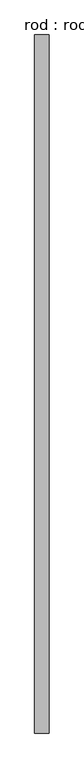
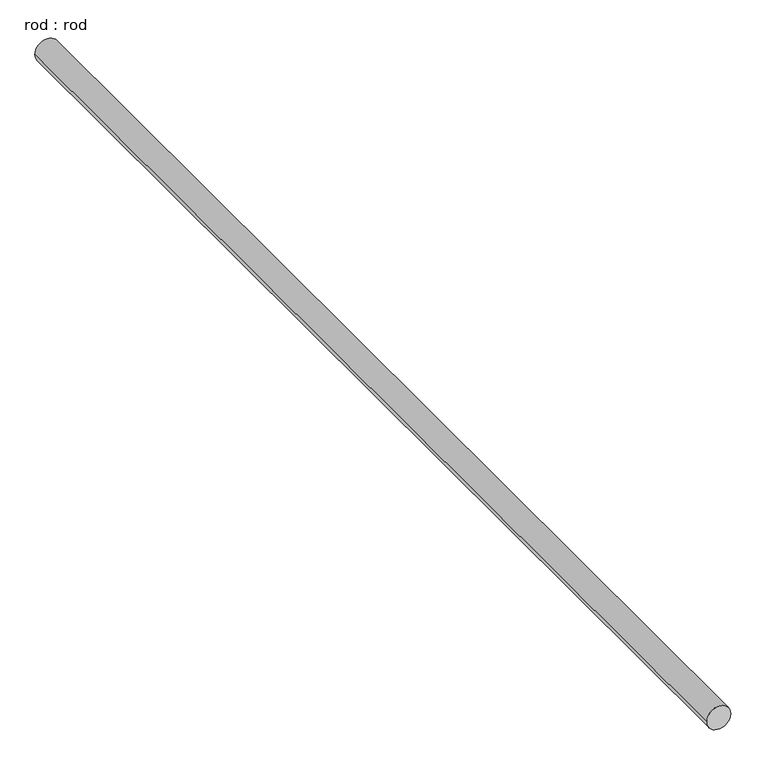
"""IFC4 building model written with IfcOpenShell, lengths in millimetres: proxy geometry, rod : rod."""

from ifc_helpers import new_model, si_unit, point, frame, frame_2d, origin, place, context, project, spatial, circle_curve, trimmed, segment, composite_curve, outline, extrude, source, transform, mapped, element, save


def rod_rod_8fd2aa88(model_context):
    return source(origin(), model_context, "Body", "SweptSolid", [
        extrude(outline(composite_curve([segment(trimmed(circle_curve(frame_2d((0.0108462, 0.0)), 200.0), [point((0.0108462, 200.0))], [point((0.0108462, -200.0))], False, "CARTESIAN"), True, "CONTINUOUS"), segment(trimmed(circle_curve(frame_2d((0.0108462, 0.0)), 200.0), [point((0.0108462, -200.0))], [point((0.0108462, 200.0))], False, "CARTESIAN"), True, "CONTINUOUS")], self_intersect=False)), frame((0.0, -5503.5844895, 0.0), z_axis=(0.0, 1.0, 0.0), x_axis=(0.0, 0.0, 1.0)), (0.0, 0.0, 1.0), 19192.6262097),
    ])


if __name__ == "__main__":
    model = new_model("IFC4")
    model_context = context("Model", 3, world=origin())
    ifc_project = project(units=[si_unit("LENGTHUNIT", "METRE", prefix="MILLI")], contexts=[model_context])
    site = spatial("IfcSite", under=ifc_project)
    building = spatial("IfcBuilding", under=site)
    placement = place(None, origin())
    rod_rod_shape = rod_rod_8fd2aa88(model_context)
    element("IfcBuildingElementProxy", 1, Name="rod : rod", ObjectType="rod : rod", at=placement, inside=building, context=model_context, shape_type="MappedRepresentation", body=[
        mapped(rod_rod_shape, transform((0.0, 0.0, 0.0), x_axis=(1.0, 0.0, 0.0), y_axis=(0.0, 1.0, 0.0), z_axis=(0.0, 0.0, 1.0))),
    ])
    save(model, "model.ifc")

# Revit data of these elements
# Type "rod : rod"
#   Default Elevation = 0
